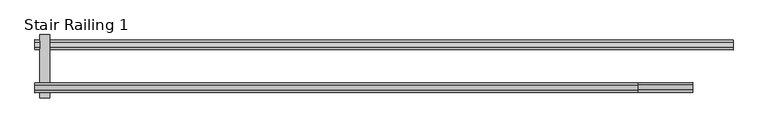
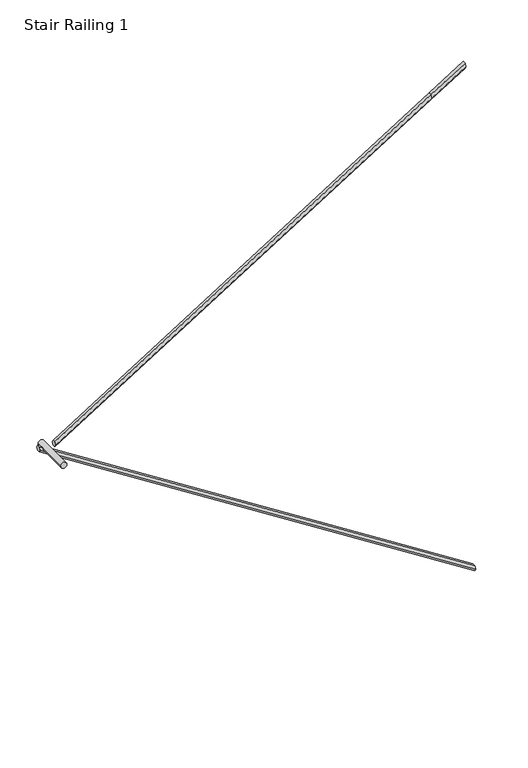
"""IFC4 building model written with IfcOpenShell, lengths in millimetres: railing geometry, Stair Railing 1."""

import ifcopenshell
import ifcopenshell.guid

model = None  # the IFC model being written
_history = None  # IfcOwnerHistory: only IFC2X3 demands one
_inside = {}  # id of a spatial element -> (the spatial element, [elements in it])
_under = {}  # id of a project, library or spatial element -> (it, [spatial elements below it])
_declared = {}  # id of a project -> (the project, [libraries it declares])
_typed = {}  # id of a type object -> (the type object, [elements of that type])
_made_of = {}  # id of a material, layer set ... -> (it, [elements and type objects made of it])


def new_model(schema):
    """Start an empty IFC model of exactly this schema.

    Asked for "IFC4X3", IfcOpenShell would pick the latest addendum, in which some entities
    have other attributes; the version numbers below select the first issue.
    IFC2X3 requires an IfcOwnerHistory on every rooted entity: one is made here for all.
    """
    global model, _history
    if schema == "IFC4X3":
        model = ifcopenshell.file(schema_version=(4, 3, 0, 0))
    else:
        model = ifcopenshell.file(schema=schema)
    _inside.clear()
    _under.clear()
    _declared.clear()
    _typed.clear()
    _made_of.clear()
    _history = None
    if model.schema == "IFC2X3":
        org = make("IfcOrganization", Name="unknown")
        user = make(
            "IfcPersonAndOrganization",
            ThePerson=make("IfcPerson", FamilyName="unknown"),
            TheOrganization=org,
        )
        app = make(
            "IfcApplication",
            ApplicationDeveloper=org,
            Version="unknown",
            ApplicationFullName="unknown",
            ApplicationIdentifier="unknown",
        )
        _history = make(
            "IfcOwnerHistory",
            OwningUser=user,
            OwningApplication=app,
            ChangeAction="ADDED",
            CreationDate=0,
        )
    return model


def make(cls, **values):
    """One entity of the class cls with the attributes given. An attribute that is None is left unset."""
    return model.create_entity(
        cls, **{name: value for name, value in values.items() if value is not None}
    )


def rooted(cls, **values):
    """An entity with a GlobalId (a new one), such as an element, a storey or a relation."""
    return make(cls, GlobalId=ifcopenshell.guid.new(), OwnerHistory=_history, **values)


def si_unit(unit_type, name, prefix=None):
    """IfcSIUnit, for example si_unit("LENGTHUNIT", "METRE", prefix="MILLI")."""
    return make("IfcSIUnit", UnitType=unit_type, Prefix=prefix, Name=name)


def assignment(units):
    """IfcUnitAssignment: the units of a project."""
    return None if units is None else make("IfcUnitAssignment", Units=units)


def point(xyz):
    """IfcCartesianPoint."""
    return None if xyz is None else make("IfcCartesianPoint", Coordinates=xyz)


def direction(xyz):
    """IfcDirection."""
    return None if xyz is None else make("IfcDirection", DirectionRatios=xyz)


def frame(location, z_axis=None, x_axis=None):
    """IfcAxis2Placement3D, a coordinate frame: its origin and axes. An axis left out is left unset."""
    return make(
        "IfcAxis2Placement3D",
        Location=point(location),
        Axis=direction(z_axis),
        RefDirection=direction(x_axis),
    )


def origin():
    """The frame at (0, 0, 0) with its axes left unset."""
    return frame((0.0, 0.0, 0.0))


def place(relative_to, where):
    """IfcLocalPlacement: puts the frame where relative to a parent placement (None: the world)."""
    return make(
        "IfcLocalPlacement", PlacementRelTo=relative_to, RelativePlacement=where
    )


def context(
    kind, dimensions, precision=None, world=None, true_north=None, identifier=None
):
    """IfcGeometricRepresentationContext, for example the 3D "Model" context."""
    return make(
        "IfcGeometricRepresentationContext",
        ContextIdentifier=identifier,
        ContextType=kind,
        CoordinateSpaceDimension=dimensions,
        Precision=precision,
        WorldCoordinateSystem=world,
        TrueNorth=true_north,
    )


def project(units=None, contexts=None):
    """IfcProject with its units and contexts."""
    return rooted(
        "IfcProject",
        Name="project",
        RepresentationContexts=contexts,
        UnitsInContext=assignment(units),
    )


def spatial(cls, under=None, at=None, **own):
    """A site, building, storey or space (cls), placed at a placement, below another one or the project."""
    s = rooted(cls, ObjectPlacement=at, **own)
    if under is not None:
        _under.setdefault(under.id(), (under, []))[1].append(s)
    return s


def circle_curve(where, radius):
    """IfcCircle in the frame where."""
    return make("IfcCircle", Position=where, Radius=radius)


def faces_of(points, faces, orient=None, outer=None):
    """IfcFace entities. A face is a list of loops; a loop is a list of indices into points, from 0.

    orient and outer hold one flag for each loop. By default every Orientation is true, the
    first loop of a face is its IfcFaceOuterBound and the others are IfcFaceBound.
    """
    made = []
    for i, loops in enumerate(faces):
        bounds = []
        for j, loop in enumerate(loops):
            is_outer = j == 0 if outer is None else outer[i][j]
            bounds.append(
                make(
                    "IfcFaceOuterBound" if is_outer else "IfcFaceBound",
                    Bound=make("IfcPolyLoop", Polygon=[points[k] for k in loop]),
                    Orientation=True if orient is None else orient[i][j],
                )
            )
        made.append(make("IfcFace", Bounds=bounds))
    return made


def faceted_brep(points, faces, orient=None, outer=None, voids=None):
    """IfcFacetedBrep: a solid bounded by flat faces; with voids (closed shells), ...WithVoids."""
    shared = [point(p) for p in points]
    hull = make("IfcClosedShell", CfsFaces=faces_of(shared, faces, orient, outer))
    if voids is None:
        return make("IfcFacetedBrep", Outer=hull)
    return make(
        "IfcFacetedBrepWithVoids",
        Outer=hull,
        Voids=[
            make(cls, CfsFaces=faces_of(shared, fs, o, b)) for cls, fs, o, b in voids
        ],
    )


def shape(context_of_items, identifier, shape_type, items):
    """IfcShapeRepresentation: the items that make up one representation, for example the "Body"."""
    return make(
        "IfcShapeRepresentation",
        ContextOfItems=context_of_items,
        RepresentationIdentifier=identifier,
        RepresentationType=shape_type,
        Items=items,
    )


def source(mapping_origin, context_of_items, identifier, shape_type, items):
    """IfcRepresentationMap: a shape defined once, which mapped items show again and again."""
    return make(
        "IfcRepresentationMap",
        MappingOrigin=mapping_origin,
        MappedRepresentation=shape(context_of_items, identifier, shape_type, items),
    )


def transform(
    local_origin,
    x_axis=None,
    y_axis=None,
    z_axis=None,
    scale=None,
    scale2=None,
    scale3=None,
    uniform=True,
):
    """IfcCartesianTransformationOperator3D, or its non-uniform kind. x_axis, y_axis, z_axis: its Axis1, 2, 3."""
    if uniform:
        return make(
            "IfcCartesianTransformationOperator3D",
            Axis1=direction(x_axis),
            Axis2=direction(y_axis),
            LocalOrigin=point(local_origin),
            Scale=scale,
            Axis3=direction(z_axis),
        )
    return make(
        "IfcCartesianTransformationOperator3DnonUniform",
        Axis1=direction(x_axis),
        Axis2=direction(y_axis),
        LocalOrigin=point(local_origin),
        Scale=scale,
        Axis3=direction(z_axis),
        Scale2=scale2,
        Scale3=scale3,
    )


def mapped(mapping_source, mapping_target):
    """IfcMappedItem: shows the shape of a source again, moved by a transform."""
    return make(
        "IfcMappedItem", MappingSource=mapping_source, MappingTarget=mapping_target
    )


def made_of(thing, what):
    """Note that an element or type object is made of a material, layer set ...; save() writes the relation."""
    if what is not None:
        _made_of.setdefault(what.id(), (what, []))[1].append(thing)
    return thing


def element(
    cls,
    number,
    at=None,
    inside=None,
    cuts=None,
    type_object=None,
    material=None,
    context=None,
    identifier="Body",
    shape_type=None,
    held_by="IfcProductDefinitionShape",
    body=None,
    shapes=None,
    **own,
):
    """One element of the class cls, such as IfcWall. Its Tag is "e" and its number.

    at: its placement. inside: the storey or other place that contains it. cuts: it is an
    opening in that element (IfcRelVoidsElement). A single representation is given by context,
    identifier, shape_type and body (its items); several are given by shapes. held_by: the class
    of the entity that holds the representations. save() writes the other relations.
    """
    e = rooted(cls, Tag="e%d" % number, ObjectPlacement=at, **own)
    if body is not None:
        shapes = [shape(context, identifier, shape_type, body)]
    if shapes is not None:
        e.Representation = make(held_by, Representations=shapes)
    if inside is not None:
        _inside.setdefault(inside.id(), (inside, []))[1].append(e)
    if cuts is not None:
        rooted(
            "IfcRelVoidsElement", RelatingBuildingElement=cuts, RelatedOpeningElement=e
        )
    if type_object is not None:
        _typed.setdefault(type_object.id(), (type_object, []))[1].append(e)
    return made_of(e, material)


def aggregate(whole, parts):
    """IfcRelAggregates: a whole, such as a stair, and the parts it consists of."""
    return rooted("IfcRelAggregates", RelatingObject=whole, RelatedObjects=parts)


def save(model, path):
    """Write the relations noted so far, then the file.

    IfcRelAggregates (storeys below a building ...), IfcRelContainedInSpatialStructure (elements
    in a storey), IfcRelDefinesByType, IfcRelAssociatesMaterial and IfcRelDeclares: one each for
    every whole, place, type object, material and project.
    """
    for whole, parts in _under.values():
        aggregate(whole, parts)
    for where, things in _inside.values():
        rooted(
            "IfcRelContainedInSpatialStructure",
            RelatedElements=things,
            RelatingStructure=where,
        )
    for kind, things in _typed.values():
        rooted("IfcRelDefinesByType", RelatedObjects=things, RelatingType=kind)
    for what, things in _made_of.values():
        rooted("IfcRelAssociatesMaterial", RelatedObjects=things, RelatingMaterial=what)
    for by, libraries in _declared.values():
        rooted("IfcRelDeclares", RelatingContext=by, RelatedDefinitions=libraries)
    model.write(path)


def plane_surface(at):
    """IfcPlane: the flat surface through the origin of the frame at, square to its z axis."""
    return make("IfcPlane", Position=at)


def cylinder_surface(at, radius):
    """IfcCylindricalSurface: all points at the distance radius from the z axis of the frame at."""
    return make("IfcCylindricalSurface", Position=at, Radius=radius)


def advanced_brep(points, edges, surfaces, faces):
    """IfcAdvancedBrep: a solid bounded by faces that lie on surfaces and meet in shared edges.

    An edge is (start, end): straight between two places in points (the first is 0);
    or (start, end, curve); or (start, end, curve, False) where it runs against its curve.
    A face is (place in surfaces, loops), or (place, loops, False) where it looks against
    its surface's normal. A loop lists edges by number (the first is 1), with a minus sign
    where the edge is run from its end to its start. The first loop is the outer one.
    """
    corners = [point(p) for p in points]
    vertices = [make("IfcVertexPoint", VertexGeometry=c) for c in corners]
    made = []
    for start, end, *more in edges:
        made.append(
            make(
                "IfcEdgeCurve",
                EdgeStart=vertices[start],
                EdgeEnd=vertices[end],
                EdgeGeometry=more[0] if more else make("IfcPolyline", Points=[corners[start], corners[end]]),
                SameSense=more[1] if len(more) > 1 else True,
            )
        )
    hull = []
    for where, loops, *sense in faces:
        bounds = []
        for j, loop in enumerate(loops):
            ring = [make("IfcOrientedEdge", EdgeElement=made[abs(k) - 1], Orientation=k > 0) for k in loop]
            bounds.append(
                make(
                    "IfcFaceOuterBound" if j == 0 else "IfcFaceBound",
                    Bound=make("IfcEdgeLoop", EdgeList=ring),
                    Orientation=True,
                )
            )
        hull.append(make("IfcAdvancedFace", Bounds=bounds, FaceSurface=surfaces[where], SameSense=sense[0] if sense else True))
    return make("IfcAdvancedBrep", Outer=make("IfcClosedShell", CfsFaces=hull))


def stair_railing_1_04a2c75b(model_context):
    return source(origin(), model_context, "Body", "SolidModel", [
        faceted_brep([(46975.6613811, 46191.4865351, 13752.6888889), (46975.6613811, 46204.1865351, 13774.6859341), (46975.6613811, 46229.5865351, 13774.6859341), (46975.6613811, 46242.2865351, 13752.6888889), (46975.6613811, 46229.5865351, 13730.6918436), (46975.6613811, 46204.1865351, 13730.6918436), (50534.1355635, 46191.4865351, 11477.9777778), (50534.1355635, 46204.1865351, 11455.9807325), (50534.1355635, 46229.5865351, 11455.9807325), (50534.1355635, 46242.2865351, 11477.9777778), (50534.1355635, 46229.5865351, 11499.974823), (50534.1355635, 46204.1865351, 11499.974823)], [[[0, 1, 2, 3, 4, 5]], [[6, 7, 8, 9, 10, 11]], [[1, 0, 6, 11]], [[2, 1, 11, 10]], [[3, 2, 10, 9]], [[4, 3, 9, 8]], [[5, 4, 8, 7]], [[0, 5, 7, 6]]]),
        advanced_brep(
        [(47051.8613811, 45946.4030566, 13752.6888889), (47001.0613811, 45946.4030566, 13752.6888889), (47051.8613811, 46267.6865351, 13752.6888889), (47001.0613811, 46267.6865351, 13752.6888889)],
        [
            (0, 1, circle_curve(frame((47026.4613811, 45946.4030566, 13752.6888889), z_axis=(0.0, -1.0, 0.0), x_axis=(1.0, 0.0, 0.0)), 25.4)),
            (1, 0, circle_curve(frame((47026.4613811, 45946.4030566, 13752.6888889), z_axis=(0.0, -1.0, 0.0), x_axis=(1.0, 0.0, 0.0)), 25.4)),
            (2, 3, circle_curve(frame((47026.4613811, 46267.6865351, 13752.6888889), z_axis=(0.0, 1.0, 0.0), x_axis=(1.0, 0.0, 0.0)), 25.4)),
            (3, 2, circle_curve(frame((47026.4613811, 46267.6865351, 13752.6888889), z_axis=(0.0, 1.0, 0.0), x_axis=(1.0, 0.0, 0.0)), 25.4)),
            (0, 2),
            (3, 1),
        ],
        [
            plane_surface(frame((47051.8613811, 45946.4030566, 13727.2888889), z_axis=(0.0, -1.0, 0.0), x_axis=(0.0, 0.0, -1.0))),
            plane_surface(frame((47051.8613811, 46267.6865351, 13727.2888889), z_axis=(0.0, 1.0, 0.0), x_axis=(0.0, 0.0, 1.0))),
            cylinder_surface(frame((47026.4613811, 46267.6865351, 13752.6888889), z_axis=(0.0, -1.0, 0.0), x_axis=(1.0, 0.0, 0.0)), 25.4),
        ],
        [
            (0, [[1, 2]]),
            (1, [[3, 4]]),
            (2, [[-1, 5, -4, 6]]),
            (2, [[-2, -6, -3, -5]]),
        ],
    ),
        faceted_brep([(50049.0613811, 46022.6030566, 15852.4222222), (50049.0613811, 46009.9030566, 15874.4192675), (50049.0613811, 45984.5030566, 15874.4192675), (50049.0613811, 45971.8030566, 15852.4222222), (50049.0613811, 45984.5030566, 15830.425177), (50049.0613811, 46009.9030566, 15830.425177), (46975.6613811, 46022.6030566, 13927.6666667), (46975.6613811, 46009.9030566, 13905.6696214), (46975.6613811, 45984.5030566, 13905.6696214), (46975.6613811, 45971.8030566, 13927.6666667), (46975.6613811, 45984.5030566, 13949.6637119), (46975.6613811, 46009.9030566, 13949.6637119)], [[[0, 1, 2, 3, 4, 5]], [[6, 7, 8, 9, 10, 11]], [[1, 0, 6, 11]], [[2, 1, 11, 10]], [[3, 2, 10, 9]], [[4, 3, 9, 8]], [[5, 4, 8, 7]], [[0, 5, 7, 6]]]),
        faceted_brep([(50328.4613811, 46022.6030566, 16027.4), (50328.4613811, 46009.9030566, 16049.3970453), (50328.4613811, 45984.5030566, 16049.3970453), (50328.4613811, 45971.8030566, 16027.4), (50328.4613811, 45984.5030566, 16005.4029547), (50328.4613811, 46009.9030566, 16005.4029547), (50049.0613811, 46022.6030566, 15852.4222222), (50049.0613811, 46009.9030566, 15830.425177), (50049.0613811, 45984.5030566, 15830.425177), (50049.0613811, 45971.8030566, 15852.4222222), (50049.0613811, 45984.5030566, 15874.4192675), (50049.0613811, 46009.9030566, 15874.4192675)], [[[0, 1, 2, 3, 4, 5]], [[6, 7, 8, 9, 10, 11]], [[1, 0, 6, 11]], [[2, 1, 11, 10]], [[3, 2, 10, 9]], [[4, 3, 9, 8]], [[5, 4, 8, 7]], [[0, 5, 7, 6]]]),
    ])


if __name__ == "__main__":
    model = new_model("IFC4")
    model_context = context("Model", 3, world=origin())
    ifc_project = project(units=[si_unit("LENGTHUNIT", "METRE", prefix="MILLI")], contexts=[model_context])
    site = spatial("IfcSite", under=ifc_project)
    building = spatial("IfcBuilding", under=site)
    placement = place(None, origin())
    stair_railing_1_shape = stair_railing_1_04a2c75b(model_context)
    element("IfcRailing", 1, ObjectType="Stair Railing 1", at=placement, inside=building, context=model_context, shape_type="MappedRepresentation", body=[
        mapped(stair_railing_1_shape, transform((0.0, 0.0, 0.0), x_axis=(1.0, 0.0, 0.0), y_axis=(0.0, 1.0, 0.0), z_axis=(0.0, 0.0, 1.0))),
    ])
    save(model, "model.ifc")

# Revit data of these elements
# Project information
#   Project Issue Date = "Issue Date"
#   Project Status = "Project Status"
#   Client Name = "Owner"
#   Project Address = "Enter address here"
#   Project Name = "Project Name"
#   Project Number = "Project Number"
